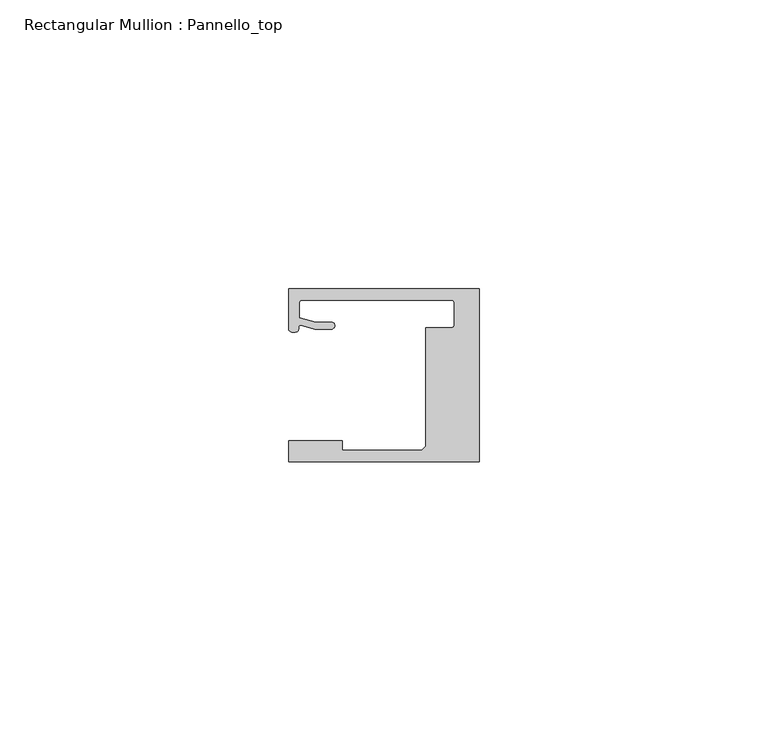
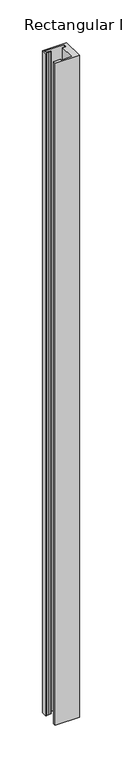
"""IFC4 building model written with IfcOpenShell, lengths in millimetres: member geometry, Rectangular Mullion : Pannello_top."""

from ifc_helpers import new_model, si_unit, frame, origin, place, context, project, spatial, polyline, circle_curve, source, transform, mapped, element, save
from ifc_brep_helpers import plane_surface, cylinder_surface, revolved_surface, extruded_surface, spline_curve, advanced_brep


def rectangular_mullion_pannello_top_b44bcb32(model_context):
    return source(origin(), model_context, "Body", "AdvancedBrep", [
        advanced_brep(
        [(-33.0, -15.0, 0.0), (0.0, -15.0, 0.0), (0.0, 15.0, 0.0), (-33.0000135, 15.0, 0.0), (-33.0000135, 8.0000472, 0.0), (-30.9223017, 8.6490241, 0.0), (-28.4999305, 7.9999523, 0.0), (-25.59998, 7.9999523, 0.0), (-25.59998, 9.1999523, 0.0), (-28.3419477, 9.1999523, 0.0), (-31.19998, 9.9657591, 0.0), (-31.19998, 12.50001, 0.0), (-30.69998, 13.00001, 0.0), (-4.7999726, 13.00001, 0.0), (-4.2999726, 12.50001, 0.0), (-4.2999726, 8.7500595, 0.0), (-4.7999726, 8.2500595, 0.0), (-9.2999726, 8.2500595, 0.0), (-9.2999726, -12.2999849, 0.0), (-10.0000103, -13.0000004, 0.0), (-23.700041, -13.0000004, 0.0), (-23.700041, -11.3000004, 0.0), (-33.0, -11.3000004, 0.0), (-33.0, -15.0, -950.0), (-33.0, -11.3000004, -950.0), (-23.700041, -11.3000004, -950.0), (-23.700041, -13.0000004, -950.0), (-10.0000103, -13.0000004, -950.0), (-9.2999726, -12.2999849, -950.0), (-9.2999726, 8.2500595, -950.0), (-4.7999726, 8.2500595, -950.0), (-4.2999726, 8.7500595, -950.0), (-4.2999726, 12.50001, -950.0), (-4.7999726, 13.00001, -950.0), (-30.69998, 13.00001, -950.0), (-31.19998, 12.50001, -950.0), (-31.19998, 9.9657591, -950.0), (-28.3419477, 9.1999523, -950.0), (-25.59998, 9.1999523, -950.0), (-25.59998, 7.9999523, -950.0), (-28.4999305, 7.9999523, -950.0), (-30.9223017, 8.6490241, -950.0), (-33.0000135, 8.0000472, -950.0), (-33.0000135, 15.0, -950.0), (0.0, 15.0, -950.0), (0.0, -15.0, -950.0)],
        [
            (0, 1),
            (1, 2),
            (2, 3),
            (3, 4),
            (4, 5, spline_curve(3, [(-33.0000135, 8.0000472, 0.0), (-33.0000135, 7.457047519, 0.0), (-32.262327879, 7.456527435, 0.0), (-31.357433266, 7.563996614, 0.0), (-31.305645054, 7.690065204, 0.0), (-31.298563602, 8.366228555, 0.0), (-31.312054066, 8.717747958, 0.0), (-30.9223017, 8.6490241, 0.0)], [4, 2, 2, 4], [0.0, 0.0027053965905959043, 0.0058611956533709, 0.007702013405570312])),
            (5, 6),
            (6, 7),
            (7, 8, circle_curve(frame((-25.59998, 8.5999523, 0.0), z_axis=(0.0, 0.0, 1.0), x_axis=(0.0, 1.0, 0.0)), 0.6)),
            (8, 9),
            (9, 10),
            (10, 11),
            (11, 12, circle_curve(frame((-30.69998, 12.50001, 0.0), z_axis=(0.0, 0.0, -1.0), x_axis=(0.0, 1.0, 0.0)), 0.5)),
            (12, 13),
            (13, 14, circle_curve(frame((-4.7999726, 12.50001, 0.0), z_axis=(0.0, 0.0, -1.0), x_axis=(1.0, 0.0, 0.0)), 0.5)),
            (14, 15),
            (15, 16, circle_curve(frame((-4.7999726, 8.7500595, 0.0), z_axis=(0.0, 0.0, -1.0), x_axis=(0.0, -1.0, 0.0)), 0.5)),
            (16, 17),
            (17, 18),
            (18, 19),
            (19, 20),
            (20, 21),
            (21, 22),
            (22, 0),
            (23, 24),
            (24, 25),
            (25, 26),
            (26, 27),
            (27, 28),
            (28, 29),
            (29, 30),
            (30, 31, circle_curve(frame((-4.7999726, 8.7500595, -950.0), z_axis=(0.0, 0.0, 1.0), x_axis=(0.0, -1.0, 0.0)), 0.5)),
            (31, 32),
            (32, 33, circle_curve(frame((-4.7999726, 12.50001, -950.0), z_axis=(0.0, 0.0, 1.0), x_axis=(1.0, 0.0, 0.0)), 0.5)),
            (33, 34),
            (34, 35, circle_curve(frame((-30.69998, 12.50001, -950.0), z_axis=(0.0, 0.0, 1.0), x_axis=(0.0, 1.0, 0.0)), 0.5)),
            (35, 36),
            (36, 37),
            (37, 38),
            (38, 39, circle_curve(frame((-25.59998, 8.5999523, -950.0), z_axis=(0.0, 0.0, -1.0), x_axis=(0.0, 1.0, 0.0)), 0.6)),
            (39, 40),
            (40, 41),
            (41, 42, spline_curve(3, [(-30.9223017, 8.6490241, -950.0), (-31.312054066, 8.717747958, -950.0), (-31.298563602, 8.366228555, -950.0), (-31.305645054, 7.690065204, -950.0), (-31.357433266, 7.563996614, -950.0), (-32.262327879, 7.456527435, -950.0), (-33.0000135, 7.457047519, -950.0), (-33.0000135, 8.0000472, -950.0)], [4, 2, 2, 4], [0.0, 0.001840817752199412, 0.004996616814974408, 0.007702013405570312])),
            (42, 43),
            (43, 44),
            (44, 45),
            (45, 23),
            (0, 23),
            (45, 1),
            (44, 2),
            (43, 3),
            (42, 4),
            (41, 5),
            (40, 6),
            (39, 7),
            (38, 8),
            (37, 9),
            (36, 10),
            (35, 11),
            (34, 12),
            (33, 13),
            (32, 14),
            (31, 15),
            (30, 16),
            (29, 17),
            (28, 18),
            (27, 19),
            (26, 20),
            (25, 21),
            (24, 22),
        ],
        [
            plane_surface(frame((0.0, -36.2491502, 0.0), z_axis=(0.0, 0.0, 1.0), x_axis=(-1.0, 0.0, 0.0))),
            plane_surface(frame((0.0, -36.2491502, -950.0), z_axis=(0.0, 0.0, -1.0), x_axis=(-1.0, 0.0, 0.0))),
            plane_surface(frame((-33.0, -15.0, 0.0), z_axis=(0.0, -1.0, 0.0), x_axis=(0.0, 0.0, -1.0))),
            plane_surface(frame((0.0, -15.0, 0.0), z_axis=(1.0, 0.0, 0.0), x_axis=(0.0, 0.0, -1.0))),
            plane_surface(frame((0.0, 15.0, 0.0), z_axis=(0.0, 1.0, 0.0), x_axis=(0.0, 0.0, -1.0))),
            plane_surface(frame((-33.0000135, 15.0, 0.0), z_axis=(-1.0, 0.0, 0.0), x_axis=(0.0, 0.0, -1.0))),
            extruded_surface(spline_curve(3, [(-33.0000135, 8.0000472, -950.0), (-33.0000135, 7.457047519, -950.0), (-32.262327879, 7.456527435, -950.0), (-31.357433266, 7.563996614, -950.0), (-31.305645054, 7.690065204, -950.0), (-31.298563602, 8.366228555, -950.0), (-31.312054066, 8.717747958, -950.0), (-30.9223017, 8.6490241, -950.0)], [4, 2, 2, 4], [0.0, 0.0027053965905959043, 0.0058611956533709, 0.007702013405570312]), (0.0, 0.0, 950.0), 950.0),
            plane_surface(frame((-30.9223017, 8.6490241, 0.0), z_axis=(-0.25881883200192934, -0.9659258833891746, 0.0), x_axis=(0.0, 0.0, -1.0))),
            plane_surface(frame((-28.4999305, 7.9999523, 0.0), z_axis=(0.0, -1.0, 0.0), x_axis=(0.0, 0.0, -1.0))),
            cylinder_surface(frame((-25.59998, 8.5999523, 0.0), z_axis=(0.0, 0.0, 1.0), x_axis=(0.0, 1.0, 0.0)), 0.6),
            plane_surface(frame((-25.59998, 9.1999523, 0.0), z_axis=(0.0, 1.0, 0.0), x_axis=(0.0, 0.0, -1.0))),
            plane_surface(frame((-28.3419477, 9.1999523, 0.0), z_axis=(0.25881883204288636, 0.9659258833782002, 0.0), x_axis=(0.0, 0.0, -1.0))),
            plane_surface(frame((-31.19998, 9.9657591, 0.0), z_axis=(1.0, 0.0, 0.0), x_axis=(0.0, 0.0, -1.0))),
            revolved_surface(polyline([(-30.69998, 13.00001, -950.0), (-30.69998, 13.00001, 0.0)]), (-30.69998, 12.50001, 0.0), (0.0, 0.0, -1.0)),
            plane_surface(frame((-30.69998, 13.00001, 0.0), z_axis=(0.0, -1.0, 0.0), x_axis=(0.0, 0.0, -1.0))),
            revolved_surface(polyline([(-4.2999726, 12.50001, -950.0), (-4.2999726, 12.50001, 0.0)]), (-4.7999726, 12.50001, 0.0), (0.0, 0.0, -1.0)),
            plane_surface(frame((-4.2999726, 12.50001, 0.0), z_axis=(-1.0, 0.0, 0.0), x_axis=(0.0, 0.0, -1.0))),
            revolved_surface(polyline([(-4.7999726, 8.2500595, -950.0), (-4.7999726, 8.2500595, 0.0)]), (-4.7999726, 8.7500595, 0.0), (0.0, 0.0, -1.0)),
            plane_surface(frame((-4.7999726, 8.2500595, 0.0), z_axis=(0.0, 1.0, 0.0), x_axis=(0.0, 0.0, -1.0))),
            plane_surface(frame((-9.2999726, 8.2500595, 0.0), z_axis=(-1.0, 0.0, 0.0), x_axis=(0.0, 0.0, -1.0))),
            plane_surface(frame((-9.2999726, -12.2999849, 0.0), z_axis=(-0.7070955486277984, 0.7071180135668678, 0.0), x_axis=(0.0, 0.0, -1.0))),
            plane_surface(frame((-10.0000103, -13.0000004, 0.0), z_axis=(0.0, 1.0, 0.0), x_axis=(0.0, 0.0, -1.0))),
            plane_surface(frame((-23.700041, -13.0000004, 0.0), z_axis=(1.0, 0.0, 0.0), x_axis=(0.0, 0.0, -1.0))),
            plane_surface(frame((-23.700041, -11.3000004, 0.0), z_axis=(0.0, 1.0, 0.0), x_axis=(0.0, 0.0, -1.0))),
            plane_surface(frame((-33.0, -11.3000004, 0.0), z_axis=(-1.0, 0.0, 0.0), x_axis=(0.0, 0.0, -1.0))),
        ],
        [
            (0, [[1, 2, 3, 4, 5, 6, 7, 8, 9, 10, 11, 12, 13, 14, 15, 16, 17, 18, 19, 20, 21, 22, 23]]),
            (1, [[24, 25, 26, 27, 28, 29, 30, 31, 32, 33, 34, 35, 36, 37, 38, 39, 40, 41, 42, 43, 44, 45, 46]]),
            (2, [[-1, 47, -46, 48]]),
            (3, [[-2, -48, -45, 49]]),
            (4, [[-3, -49, -44, 50]]),
            (5, [[-4, -50, -43, 51]]),
            (6, [[-5, -51, -42, 52]]),
            (7, [[-6, -52, -41, 53]]),
            (8, [[-7, -53, -40, 54]]),
            (9, [[-8, -54, -39, 55]]),
            (10, [[-9, -55, -38, 56]]),
            (11, [[-10, -56, -37, 57]]),
            (12, [[-11, -57, -36, 58]]),
            (13, [[-12, -58, -35, 59]]),
            (14, [[-13, -59, -34, 60]]),
            (15, [[-14, -60, -33, 61]]),
            (16, [[-15, -61, -32, 62]]),
            (17, [[-16, -62, -31, 63]]),
            (18, [[-17, -63, -30, 64]]),
            (19, [[-18, -64, -29, 65]]),
            (20, [[-19, -65, -28, 66]]),
            (21, [[-20, -66, -27, 67]]),
            (22, [[-21, -67, -26, 68]]),
            (23, [[-22, -68, -25, 69]]),
            (24, [[-23, -69, -24, -47]]),
        ],
    ),
    ])


if __name__ == "__main__":
    model = new_model("IFC4")
    model_context = context("Model", 3, world=origin())
    ifc_project = project(units=[si_unit("LENGTHUNIT", "METRE", prefix="MILLI")], contexts=[model_context])
    site = spatial("IfcSite", under=ifc_project)
    building = spatial("IfcBuilding", under=site)
    placement = place(None, origin())
    rectangular_mullion_pannello_top_shape = rectangular_mullion_pannello_top_b44bcb32(model_context)
    element("IfcMember", 1, ObjectType="Rectangular Mullion : Pannello_top", at=placement, inside=building, context=model_context, shape_type="MappedRepresentation", body=[
        mapped(rectangular_mullion_pannello_top_shape, transform((0.0, 0.0, 0.0), x_axis=(1.0, 0.0, 0.0), y_axis=(0.0, 1.0, 0.0), z_axis=(0.0, 0.0, 1.0))),
    ])
    save(model, "model.ifc")

# Revit data of these elements
# Type "Rectangular Mullion : Pannello_top"
#   built-in parameter 1007322 = 0.0984252 (stored number, unit not read)
#   built-in parameter 1007321 = 0 (stored number, unit not read)
#   built-in parameter 1007320 = 0.0305117 (stored number, unit not read)
